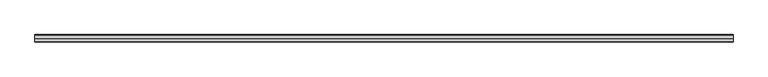
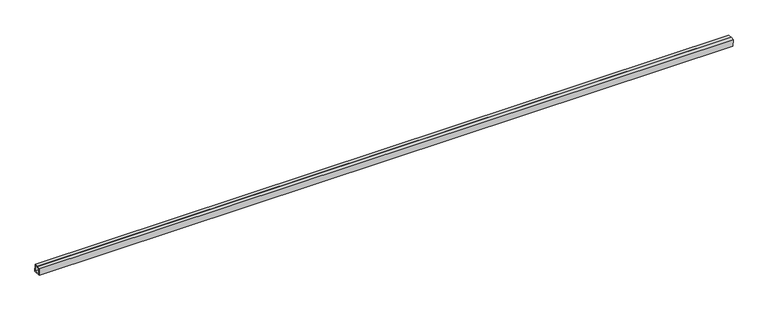
"""IFC4 building model written with IfcOpenShell, lengths in millimetres: proxy geometry, Inner panel:Inner panel:1:Inner panel:1 : Inner panel:Inner panel:300324:2:Inner panel:1:Inner panel:1 : Inner panel:Inner panel:300324:2 : Inner panel:Inner panel:1:Inner panel:1 : Inner panel:Inner panel:300324:300043:51 : Inner panel:Inner panel:1:Inner panel:1 : Inner panel:Inner panel:300324:2:Inner panel:1:Inner panel:1 : Inner panel:Inner panel:300324:2 : Inner panel:Inner panel:1:Inner panel:1 : Inner panel:Inner panel:300324:300043:308120."""

from ifc_helpers import new_model, si_unit, frame, origin, place, context, project, spatial, polyline, outline, extrude, source, transform, mapped, element, save


def generic_models_551d77a5(model_context):
    return source(origin(), model_context, "Body", "SweptSolid", [
        extrude(outline(polyline([(-578476.5317668, 3971.7383355), (-578458.2913437, 3972.4983531), (-578456.7052199, 3934.431383), (-578494.77219, 3932.8452593), (-578496.3583138, 3970.9122294), (-578478.1178906, 3971.672247), (-578478.0187579, 3969.2930614), (-578493.8799954, 3968.6321765), (-578492.4921371, 3935.3235776), (-578459.1835383, 3936.7114359), (-578460.5713966, 3970.0200347), (-578476.4326341, 3969.3591498), (-578476.5317668, 3971.7383355)])), frame((664223.0867238, 0.0, 0.0), z_axis=(1.0, 0.0, 0.0), x_axis=(0.0, 1.0, 0.0)), (0.0, 0.0, 1.0), 3657.6),
    ])


if __name__ == "__main__":
    model = new_model("IFC4")
    model_context = context("Model", 3, world=origin())
    ifc_project = project(units=[si_unit("LENGTHUNIT", "METRE", prefix="MILLI")], contexts=[model_context])
    site = spatial("IfcSite", under=ifc_project)
    building = spatial("IfcBuilding", under=site)
    placement = place(None, origin())
    generic_models_shape = generic_models_551d77a5(model_context)
    element("IfcBuildingElementProxy", 1, Name="Inner panel:Inner panel:1:Inner panel:1 : Inner panel:Inner panel:300324:2:Inner panel:1:Inner panel:1 : Inner panel:Inner panel:300324:2 : Inner panel:Inner panel:1:Inner panel:1 : Inner panel:Inner panel:300324:300043:51 : Inner panel:Inner panel:1:Inner panel:1 : Inner panel:Inner panel:300324:2:Inner panel:1:Inner panel:1 : Inner panel:Inner panel:300324:2 : Inner panel:Inner panel:1:Inner panel:1 : Inner panel:Inner panel:300324:300043:308120", ObjectType="Inner panel:Inner panel:1:Inner panel:1 : Inner panel:Inner panel:300324:2:Inner panel:1:Inner panel:1 : Inner panel:Inner panel:300324:2 : Inner panel:Inner panel:1:Inner panel:1 : Inner panel:Inner panel:300324:300043:51 : Inner panel:Inner panel:1:Inner panel:1 : Inner panel:Inner panel:300324:2:Inner panel:1:Inner panel:1 : Inner panel:Inner panel:300324:2 : Inner panel:Inner panel:1:Inner panel:1 : Inner panel:Inner panel:300324:300043:308120", at=placement, inside=building, context=model_context, shape_type="MappedRepresentation", body=[
        mapped(generic_models_shape, transform((0.0, 0.0, 0.0), x_axis=(1.0, 0.0, 0.0), y_axis=(0.0, 1.0, 0.0), z_axis=(0.0, 0.0, 1.0))),
    ])
    save(model, "model.ifc")

# Revit data of these elements
# Type "Inner panel:Inner panel:1:Inner panel:1 : Inner panel:Inner panel:300324:2:Inner panel:1:Inner panel:1 : Inner panel:Inner panel:300324:2 : Inner panel:Inner panel:1:Inner panel:1 : Inner panel:Inner panel:300324:300043:51 : Inner panel:Inner panel:1:Inner panel:1 : Inner panel:Inner panel:300324:2:Inner panel:1:Inner panel:1 : Inner panel:Inner panel:300324:2 : Inner panel:Inner panel:1:Inner panel:1 : Inner panel:Inner panel:300324:300043:308120"
#   NameOverride = "Inner panel:Inner panel:1:Inner panel:1 : Inner panel:Inner panel:300324:2:Inner panel:1:Inner panel:1 : Inner panel:Inner panel:300324:2 : Inner panel:Inner panel:1:Inner panel:1 : Inner panel:Inner panel:300324:300043:308120"
#   ObjectTypeOverride = "Inner panel:1:Inner panel:1 : Inner panel:Inner panel:300324:2 : Inner panel:Inner panel:1:Inner panel:1 : Inner panel:Inner panel:300324:300043"
#   Reference = "Inner panel"
#   Tag = "308120"
# Element 1 (IfcBuildingElementProxy, "Inner panel:Inner panel:1:Inner panel:1 : Inner panel:Inner panel:300324:2:Inner panel:1:Inner panel:1 : Inner panel:Inner panel:300324:2 : Inner panel:Inner panel:1:Inner panel:1 : Inner panel:Inner panel:300324:300043:51 : Inner panel:Inner panel:1:Inner panel:1 : Inner panel:Inner panel:300324:2:Inner panel:1:Inner panel:1 : Inner panel:Inner panel:300324:2 : Inner panel:Inner panel:1:Inner panel:1 : Inner panel:Inner panel:300324:300043:308120")
#   Materials on its faces: "1 1/2\" X 1 1/2\" SPLIT-SEAM SQUARE TUBING (~24\" CANTILEVER FROM C.L. OF GLULAM)"
# Materials
#   "1 1/2\" X 1 1/2\" SPLIT-SEAM SQUARE TUBING (~24\" CANTILEVER FROM C.L. OF GLULAM)": class "Unassigned", colour RGB 202 201 200, transparency 0, Cost = 0
